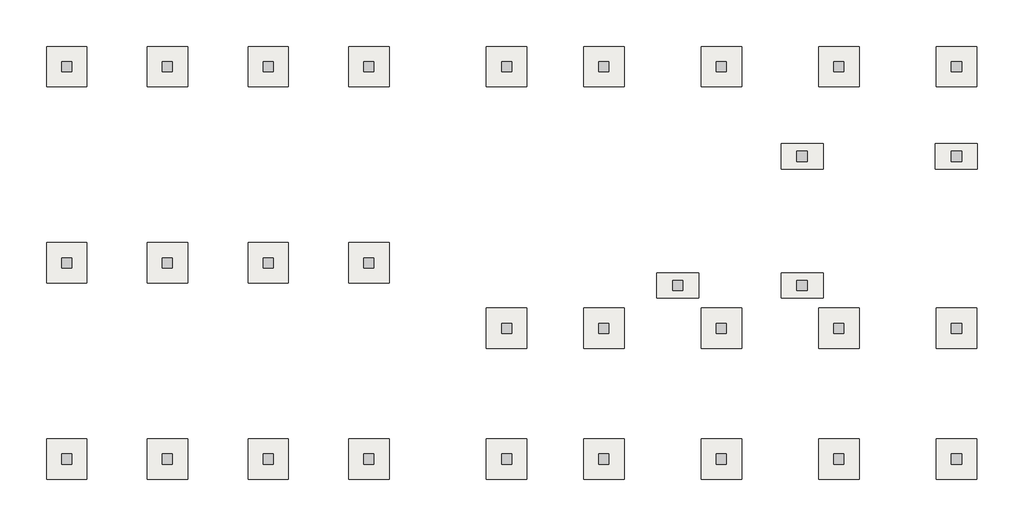
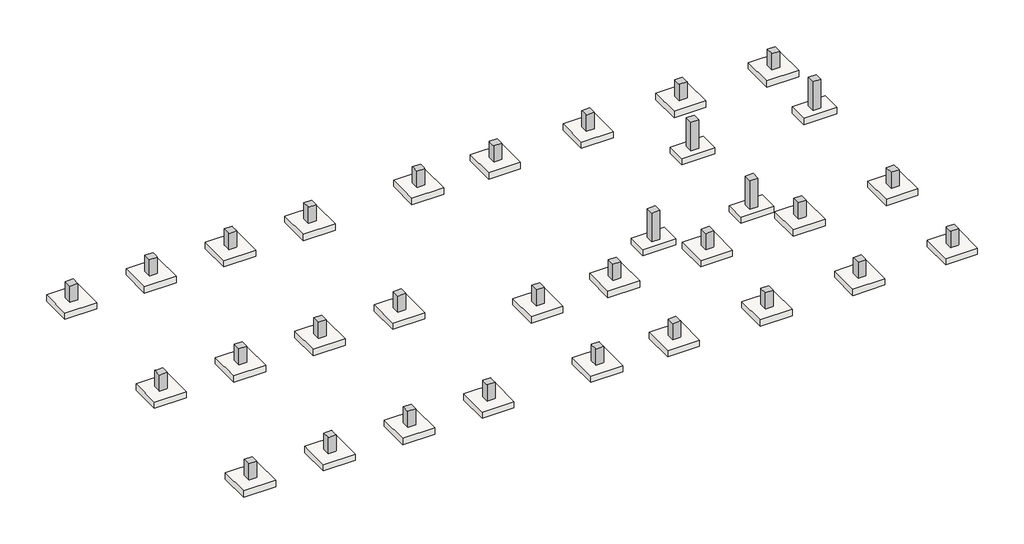
# Not in any storey: 31 columns, 31 slabs.
"""IFC4 building model written with IfcOpenShell, lengths in millimetres."""

import ifcopenshell
import ifcopenshell.guid

model = None  # the IFC model being written
_history = None  # IfcOwnerHistory: only IFC2X3 demands one
_inside = {}  # id of a spatial element -> (the spatial element, [elements in it])
_under = {}  # id of a project, library or spatial element -> (it, [spatial elements below it])
_declared = {}  # id of a project -> (the project, [libraries it declares])
_typed = {}  # id of a type object -> (the type object, [elements of that type])
_made_of = {}  # id of a material, layer set ... -> (it, [elements and type objects made of it])


def new_model(schema):
    """Start an empty IFC model of exactly this schema.

    Asked for "IFC4X3", IfcOpenShell would pick the latest addendum, in which some entities
    have other attributes; the version numbers below select the first issue.
    IFC2X3 requires an IfcOwnerHistory on every rooted entity: one is made here for all.
    """
    global model, _history
    if schema == "IFC4X3":
        model = ifcopenshell.file(schema_version=(4, 3, 0, 0))
    else:
        model = ifcopenshell.file(schema=schema)
    _inside.clear()
    _under.clear()
    _declared.clear()
    _typed.clear()
    _made_of.clear()
    _history = None
    if model.schema == "IFC2X3":
        org = make("IfcOrganization", Name="unknown")
        user = make(
            "IfcPersonAndOrganization",
            ThePerson=make("IfcPerson", FamilyName="unknown"),
            TheOrganization=org,
        )
        app = make(
            "IfcApplication",
            ApplicationDeveloper=org,
            Version="unknown",
            ApplicationFullName="unknown",
            ApplicationIdentifier="unknown",
        )
        _history = make(
            "IfcOwnerHistory",
            OwningUser=user,
            OwningApplication=app,
            ChangeAction="ADDED",
            CreationDate=0,
        )
    return model


def make(cls, **values):
    """One entity of the class cls with the attributes given. An attribute that is None is left unset."""
    return model.create_entity(
        cls, **{name: value for name, value in values.items() if value is not None}
    )


def rooted(cls, **values):
    """An entity with a GlobalId (a new one), such as an element, a storey or a relation."""
    return make(cls, GlobalId=ifcopenshell.guid.new(), OwnerHistory=_history, **values)


def si_unit(unit_type, name, prefix=None):
    """IfcSIUnit, for example si_unit("LENGTHUNIT", "METRE", prefix="MILLI")."""
    return make("IfcSIUnit", UnitType=unit_type, Prefix=prefix, Name=name)


def assignment(units):
    """IfcUnitAssignment: the units of a project."""
    return None if units is None else make("IfcUnitAssignment", Units=units)


def point(xyz):
    """IfcCartesianPoint."""
    return None if xyz is None else make("IfcCartesianPoint", Coordinates=xyz)


def direction(xyz):
    """IfcDirection."""
    return None if xyz is None else make("IfcDirection", DirectionRatios=xyz)


def frame(location, z_axis=None, x_axis=None):
    """IfcAxis2Placement3D, a coordinate frame: its origin and axes. An axis left out is left unset."""
    return make(
        "IfcAxis2Placement3D",
        Location=point(location),
        Axis=direction(z_axis),
        RefDirection=direction(x_axis),
    )


def origin():
    """The frame at (0, 0, 0) with its axes left unset."""
    return frame((0.0, 0.0, 0.0))


def place(relative_to, where):
    """IfcLocalPlacement: puts the frame where relative to a parent placement (None: the world)."""
    return make(
        "IfcLocalPlacement", PlacementRelTo=relative_to, RelativePlacement=where
    )


def context(
    kind, dimensions, precision=None, world=None, true_north=None, identifier=None
):
    """IfcGeometricRepresentationContext, for example the 3D "Model" context."""
    return make(
        "IfcGeometricRepresentationContext",
        ContextIdentifier=identifier,
        ContextType=kind,
        CoordinateSpaceDimension=dimensions,
        Precision=precision,
        WorldCoordinateSystem=world,
        TrueNorth=true_north,
    )


def project(units=None, contexts=None):
    """IfcProject with its units and contexts."""
    return rooted(
        "IfcProject",
        Name="project",
        RepresentationContexts=contexts,
        UnitsInContext=assignment(units),
    )


def spatial(cls, under=None, at=None, **own):
    """A site, building, storey or space (cls), placed at a placement, below another one or the project."""
    s = rooted(cls, ObjectPlacement=at, **own)
    if under is not None:
        _under.setdefault(under.id(), (under, []))[1].append(s)
    return s


def polyline(points):
    """IfcPolyline through the points."""
    return make("IfcPolyline", Points=[point(p) for p in points])


def outline(outer, holes=None, kind="AREA"):
    """IfcArbitraryClosedProfileDef: a profile drawn as a closed curve; with holes, ...WithVoids."""
    if holes is None:
        return make("IfcArbitraryClosedProfileDef", ProfileType=kind, OuterCurve=outer)
    return make(
        "IfcArbitraryProfileDefWithVoids",
        ProfileType=kind,
        OuterCurve=outer,
        InnerCurves=holes,
    )


def extrude(swept, where, along, depth):
    """IfcExtrudedAreaSolid: the profile swept, set in the frame where, extruded along a direction by depth."""
    return make(
        "IfcExtrudedAreaSolid",
        SweptArea=swept,
        Position=where,
        ExtrudedDirection=direction(along),
        Depth=depth,
    )


def faces_of(points, faces, orient=None, outer=None):
    """IfcFace entities. A face is a list of loops; a loop is a list of indices into points, from 0.

    orient and outer hold one flag for each loop. By default every Orientation is true, the
    first loop of a face is its IfcFaceOuterBound and the others are IfcFaceBound.
    """
    made = []
    for i, loops in enumerate(faces):
        bounds = []
        for j, loop in enumerate(loops):
            is_outer = j == 0 if outer is None else outer[i][j]
            bounds.append(
                make(
                    "IfcFaceOuterBound" if is_outer else "IfcFaceBound",
                    Bound=make("IfcPolyLoop", Polygon=[points[k] for k in loop]),
                    Orientation=True if orient is None else orient[i][j],
                )
            )
        made.append(make("IfcFace", Bounds=bounds))
    return made


def faceted_brep(points, faces, orient=None, outer=None, voids=None):
    """IfcFacetedBrep: a solid bounded by flat faces; with voids (closed shells), ...WithVoids."""
    shared = [point(p) for p in points]
    hull = make("IfcClosedShell", CfsFaces=faces_of(shared, faces, orient, outer))
    if voids is None:
        return make("IfcFacetedBrep", Outer=hull)
    return make(
        "IfcFacetedBrepWithVoids",
        Outer=hull,
        Voids=[
            make(cls, CfsFaces=faces_of(shared, fs, o, b)) for cls, fs, o, b in voids
        ],
    )


def shape(context_of_items, identifier, shape_type, items):
    """IfcShapeRepresentation: the items that make up one representation, for example the "Body"."""
    return make(
        "IfcShapeRepresentation",
        ContextOfItems=context_of_items,
        RepresentationIdentifier=identifier,
        RepresentationType=shape_type,
        Items=items,
    )


def source(mapping_origin, context_of_items, identifier, shape_type, items):
    """IfcRepresentationMap: a shape defined once, which mapped items show again and again."""
    return make(
        "IfcRepresentationMap",
        MappingOrigin=mapping_origin,
        MappedRepresentation=shape(context_of_items, identifier, shape_type, items),
    )


def transform(
    local_origin,
    x_axis=None,
    y_axis=None,
    z_axis=None,
    scale=None,
    scale2=None,
    scale3=None,
    uniform=True,
):
    """IfcCartesianTransformationOperator3D, or its non-uniform kind. x_axis, y_axis, z_axis: its Axis1, 2, 3."""
    if uniform:
        return make(
            "IfcCartesianTransformationOperator3D",
            Axis1=direction(x_axis),
            Axis2=direction(y_axis),
            LocalOrigin=point(local_origin),
            Scale=scale,
            Axis3=direction(z_axis),
        )
    return make(
        "IfcCartesianTransformationOperator3DnonUniform",
        Axis1=direction(x_axis),
        Axis2=direction(y_axis),
        LocalOrigin=point(local_origin),
        Scale=scale,
        Axis3=direction(z_axis),
        Scale2=scale2,
        Scale3=scale3,
    )


def mapped(mapping_source, mapping_target):
    """IfcMappedItem: shows the shape of a source again, moved by a transform."""
    return make(
        "IfcMappedItem", MappingSource=mapping_source, MappingTarget=mapping_target
    )


def made_of(thing, what):
    """Note that an element or type object is made of a material, layer set ...; save() writes the relation."""
    if what is not None:
        _made_of.setdefault(what.id(), (what, []))[1].append(thing)
    return thing


def element(
    cls,
    number,
    at=None,
    inside=None,
    cuts=None,
    type_object=None,
    material=None,
    context=None,
    identifier="Body",
    shape_type=None,
    held_by="IfcProductDefinitionShape",
    body=None,
    shapes=None,
    **own,
):
    """One element of the class cls, such as IfcWall. Its Tag is "e" and its number.

    at: its placement. inside: the storey or other place that contains it. cuts: it is an
    opening in that element (IfcRelVoidsElement). A single representation is given by context,
    identifier, shape_type and body (its items); several are given by shapes. held_by: the class
    of the entity that holds the representations. save() writes the other relations.
    """
    e = rooted(cls, Tag="e%d" % number, ObjectPlacement=at, **own)
    if body is not None:
        shapes = [shape(context, identifier, shape_type, body)]
    if shapes is not None:
        e.Representation = make(held_by, Representations=shapes)
    if inside is not None:
        _inside.setdefault(inside.id(), (inside, []))[1].append(e)
    if cuts is not None:
        rooted(
            "IfcRelVoidsElement", RelatingBuildingElement=cuts, RelatedOpeningElement=e
        )
    if type_object is not None:
        _typed.setdefault(type_object.id(), (type_object, []))[1].append(e)
    return made_of(e, material)


def aggregate(whole, parts):
    """IfcRelAggregates: a whole, such as a stair, and the parts it consists of."""
    return rooted("IfcRelAggregates", RelatingObject=whole, RelatedObjects=parts)


def save(model, path):
    """Write the relations noted so far, then the file.

    IfcRelAggregates (storeys below a building ...), IfcRelContainedInSpatialStructure (elements
    in a storey), IfcRelDefinesByType, IfcRelAssociatesMaterial and IfcRelDeclares: one each for
    every whole, place, type object, material and project.
    """
    for whole, parts in _under.values():
        aggregate(whole, parts)
    for where, things in _inside.values():
        rooted(
            "IfcRelContainedInSpatialStructure",
            RelatedElements=things,
            RelatingStructure=where,
        )
    for kind, things in _typed.values():
        rooted("IfcRelDefinesByType", RelatedObjects=things, RelatingType=kind)
    for what, things in _made_of.values():
        rooted("IfcRelAssociatesMaterial", RelatedObjects=things, RelatingMaterial=what)
    for by, libraries in _declared.values():
        rooted("IfcRelDeclares", RelatingContext=by, RelatedDefinitions=libraries)
    model.write(path)


def ft211_footing_rectangular_r1_5fe39465(model_context):
    return source(origin(), model_context, "Body", "SweptSolid", [
        extrude(outline(polyline([(1200.0, 1200.0), (1200.0, -1200.0), (-1200.0, -1200.0), (-1200.0, 1200.0), (1200.0, 1200.0)])), frame((0.0, 0.0, -500.0), z_axis=(0.0, 0.0, 1.0), x_axis=(1.0, 0.0, 0.0)), (0.0, 0.0, 1.0), 500.0),
    ])


def ft211_footing_rectangular_r1_907a7f09(model_context):
    return source(origin(), model_context, "Body", "SweptSolid", [
        extrude(outline(polyline([(1250.0, 750.0), (1250.0, -750.0), (-1250.0, -750.0), (-1250.0, 750.0), (1250.0, 750.0)])), frame((0.0, 0.0, -500.0), z_axis=(0.0, 0.0, 1.0), x_axis=(1.0, 0.0, 0.0)), (0.0, 0.0, 1.0), 500.0),
    ])


model = new_model("IFC4")

# Units and contexts
model_context = context("Model", 3, world=origin())
ifc_project = project(units=[si_unit("LENGTHUNIT", "METRE", prefix="MILLI")], contexts=[model_context])

# Site, building
site = spatial("IfcSite", under=ifc_project)
building = spatial("IfcBuilding", under=site)

# Columns
placement = place(None, origin())
element("IfcColumn", 1, ObjectType="RC_Column_Rectangular : H_SC_ACC_UG PED_W600xL600", at=placement, inside=building, context=model_context, shape_type="Brep", body=[
    faceted_brep([(224.7, 12616.5208589, -1150.0), (224.7, 12016.5208589, -1150.0), (-375.3, 12016.5208589, -1150.0), (-375.3, 12616.5208589, -1150.0), (224.7, 12616.5208589, 150.0), (224.7, 12016.5208589, 150.0), (-375.3, 12016.5208589, 150.0), (-375.3, 12616.5208589, 150.0), (-275.3, 12616.5208589, 150.0), (124.7, 12616.5208589, 150.0)], [[[0, 1, 2, 3]], [[4, 5, 1, 0]], [[5, 6, 2, 1]], [[6, 7, 3, 2]], [[7, 8, 9, 4, 0, 3]], [[4, 9, 8, 7, 6, 5]]]),
])
element("IfcColumn", 2, ObjectType="RC_Column_Rectangular : H_SC_ACC_UG PED_W600xL600", at=placement, inside=building, context=model_context, shape_type="SweptSolid", body=[
    extrude(outline(polyline([(6224.7, 12616.5208589), (6224.7, 12016.5208589), (5624.7, 12016.5208589), (5624.7, 12616.5208589), (6224.7, 12616.5208589)])), frame((0.0, 0.0, -1150.0), z_axis=(0.0, 0.0, 1.0), x_axis=(1.0, 0.0, 0.0)), (0.0, 0.0, 1.0), 1300.0),
])
element("IfcColumn", 3, ObjectType="RC_Column_Rectangular : H_SC_ACC_UG PED_W600xL600", at=placement, inside=building, context=model_context, shape_type="SweptSolid", body=[
    extrude(outline(polyline([(12224.7, 12616.5208589), (12224.7, 12016.5208589), (11624.7, 12016.5208589), (11624.7, 12616.5208589), (12224.7, 12616.5208589)])), frame((0.0, 0.0, -1150.0), z_axis=(0.0, 0.0, 1.0), x_axis=(1.0, 0.0, 0.0)), (0.0, 0.0, 1.0), 1300.0),
])
element("IfcColumn", 4, ObjectType="RC_Column_Rectangular : H_SC_ACC_UG PED_W600xL600", at=placement, inside=building, context=model_context, shape_type="SweptSolid", body=[
    extrude(outline(polyline([(18224.7, 12616.5208589), (18224.7, 12016.5208589), (17624.7, 12016.5208589), (17624.7, 12616.5208589), (18224.7, 12616.5208589)])), frame((0.0, 0.0, -1150.0), z_axis=(0.0, 0.0, 1.0), x_axis=(1.0, 0.0, 0.0)), (0.0, 0.0, 1.0), 1300.0),
])
element("IfcColumn", 5, ObjectType="RC_Column_Rectangular : H_SC_ACC_UG PED_W600xL600", at=placement, inside=building, context=model_context, shape_type="Brep", body=[
    faceted_brep([(224.7, 24316.5208589, -1150.0), (224.7, 23716.5208589, -1150.0), (-375.3, 23716.5208589, -1150.0), (-375.3, 24316.5208589, -1150.0), (224.7, 24316.5208589, 150.0), (224.7, 23716.5208589, 150.0), (124.7, 23716.5208589, 150.0), (-275.3, 23716.5208589, 150.0), (-375.3, 23716.5208589, 150.0), (-375.3, 24316.5208589, 150.0)], [[[0, 1, 2, 3]], [[4, 5, 1, 0]], [[5, 6, 7, 8, 2, 1]], [[8, 9, 3, 2]], [[9, 4, 0, 3]], [[4, 9, 8, 7, 6, 5]]]),
])
element("IfcColumn", 6, ObjectType="RC_Column_Rectangular : H_SC_ACC_UG PED_W600xL600", at=placement, inside=building, context=model_context, shape_type="Brep", body=[
    faceted_brep([(6224.7, 24316.5208589, -1150.0), (6224.7, 23716.5208589, -1150.0), (5624.7, 23716.5208589, -1150.0), (5624.7, 24316.5208589, -1150.0), (6224.7, 24316.5208589, 150.0), (6224.7, 24216.5208589, 150.0), (6224.7, 23816.5208589, 150.0), (6224.7, 23716.5208589, 150.0), (5624.7, 23716.5208589, 150.0), (5624.7, 23816.5208589, 150.0), (5624.7, 24216.5208589, 150.0), (5624.7, 24316.5208589, 150.0)], [[[0, 1, 2, 3]], [[4, 5, 6, 7, 1, 0]], [[7, 8, 2, 1]], [[8, 9, 10, 11, 3, 2]], [[11, 4, 0, 3]], [[4, 11, 10, 9, 8, 7, 6, 5]]]),
])
element("IfcColumn", 7, ObjectType="RC_Column_Rectangular : H_SC_ACC_UG PED_W600xL600", at=placement, inside=building, context=model_context, shape_type="Brep", body=[
    faceted_brep([(12224.7, 24316.5208589, -1150.0), (12224.7, 23716.5208589, -1150.0), (11624.7, 23716.5208589, -1150.0), (11624.7, 24316.5208589, -1150.0), (12224.7, 24316.5208589, 150.0), (12224.7, 24216.5208589, 150.0), (12224.7, 23816.5208589, 150.0), (12224.7, 23716.5208589, 150.0), (11624.7, 23716.5208589, 150.0), (11624.7, 23816.5208589, 150.0), (11624.7, 24216.5208589, 150.0), (11624.7, 24316.5208589, 150.0)], [[[0, 1, 2, 3]], [[4, 5, 6, 7, 1, 0]], [[7, 8, 2, 1]], [[8, 9, 10, 11, 3, 2]], [[11, 4, 0, 3]], [[4, 11, 10, 9, 8, 7, 6, 5]]]),
])
element("IfcColumn", 8, ObjectType="RC_Column_Rectangular : H_SC_ACC_UG PED_W600xL600", at=placement, inside=building, context=model_context, shape_type="Brep", body=[
    faceted_brep([(18224.7, 24316.5208589, -1150.0), (18224.7, 23716.5208589, -1150.0), (17624.7, 23716.5208589, -1150.0), (17624.7, 24316.5208589, -1150.0), (18224.7, 24316.5208589, 150.0), (18224.7, 24216.5208589, 150.0), (18224.7, 23816.5208589, 150.0), (18224.7, 23716.5208589, 150.0), (17624.7, 23716.5208589, 150.0), (17624.7, 23816.5208589, 150.0), (17624.7, 24216.5208589, 150.0), (17624.7, 24316.5208589, 150.0)], [[[0, 1, 2, 3]], [[4, 5, 6, 7, 1, 0]], [[7, 8, 2, 1]], [[8, 9, 10, 11, 3, 2]], [[11, 4, 0, 3]], [[4, 11, 10, 9, 8, 7, 6, 5]]]),
])
element("IfcColumn", 9, ObjectType="RC_Column_Rectangular : H_SC_ACC_UG PED_W600xL600", at=placement, inside=building, context=model_context, shape_type="Brep", body=[
    faceted_brep([(26424.7, 24316.5208589, -1150.0), (26424.7, 23716.5208589, -1150.0), (25824.7, 23716.5208589, -1150.0), (25824.7, 24316.5208589, -1150.0), (26424.7, 24316.5208589, 150.0), (26424.7, 24216.5208589, 150.0), (26424.7, 23816.5208589, 150.0), (26424.7, 23716.5208589, 150.0), (25824.7, 23716.5208589, 150.0), (25824.7, 23816.5208589, 150.0), (25824.7, 24216.5208589, 150.0), (25824.7, 24316.5208589, 150.0)], [[[0, 1, 2, 3]], [[4, 5, 6, 7, 1, 0]], [[7, 8, 2, 1]], [[8, 9, 10, 11, 3, 2]], [[11, 4, 0, 3]], [[4, 11, 10, 9, 8, 7, 6, 5]]]),
])
element("IfcColumn", 10, ObjectType="RC_Column_Rectangular : H_SC_ACC_UG PED_W600xL600", at=placement, inside=building, context=model_context, shape_type="Brep", body=[
    faceted_brep([(32224.7, 24316.5208589, -1150.0), (32224.7, 23716.5208589, -1150.0), (31624.7, 23716.5208589, -1150.0), (31624.7, 24316.5208589, -1150.0), (32224.7, 24316.5208589, 150.0), (32224.7, 24216.5208589, 150.0), (32224.7, 23816.5208589, 150.0), (32224.7, 23716.5208589, 150.0), (31624.7, 23716.5208589, 150.0), (31624.7, 23816.5208589, 150.0), (31624.7, 24216.5208589, 150.0), (31624.7, 24316.5208589, 150.0)], [[[0, 1, 2, 3]], [[4, 5, 6, 7, 1, 0]], [[7, 8, 2, 1]], [[8, 9, 10, 11, 3, 2]], [[11, 4, 0, 3]], [[4, 11, 10, 9, 8, 7, 6, 5]]]),
])
element("IfcColumn", 11, ObjectType="RC_Column_Rectangular : H_SC_ACC_UG PED_W600xL600", at=placement, inside=building, context=model_context, shape_type="Brep", body=[
    faceted_brep([(39224.7, 24316.5208589, -1150.0), (39224.7, 23716.5208589, -1150.0), (38624.7, 23716.5208589, -1150.0), (38624.7, 24316.5208589, -1150.0), (39224.7, 24316.5208589, 150.0), (39224.7, 24216.5208589, 150.0), (39224.7, 23816.5208589, 150.0), (39224.7, 23716.5208589, 150.0), (38624.7, 23716.5208589, 150.0), (38624.7, 23816.5208589, 150.0), (38624.7, 24216.5208589, 150.0), (38624.7, 24316.5208589, 150.0)], [[[0, 1, 2, 3]], [[4, 5, 6, 7, 1, 0]], [[7, 8, 2, 1]], [[8, 9, 10, 11, 3, 2]], [[11, 4, 0, 3]], [[4, 11, 10, 9, 8, 7, 6, 5]]]),
])
element("IfcColumn", 12, ObjectType="RC_Column_Rectangular : H_SC_ACC_UG PED_W600xL600", at=placement, inside=building, context=model_context, shape_type="Brep", body=[
    faceted_brep([(46224.7, 24316.5208589, -1150.0), (46224.7, 23716.5208589, -1150.0), (45624.7, 23716.5208589, -1150.0), (45624.7, 24316.5208589, -1150.0), (46224.7, 24316.5208589, 150.0), (46224.7, 24216.5208589, 150.0), (46224.7, 23816.5208589, 150.0), (46224.7, 23716.5208589, 150.0), (45624.7, 23716.5208589, 150.0), (45624.7, 23816.5208589, 150.0), (45624.7, 24216.5208589, 150.0), (45624.7, 24316.5208589, 150.0)], [[[0, 1, 2, 3]], [[4, 5, 6, 7, 1, 0]], [[7, 8, 2, 1]], [[8, 9, 10, 11, 3, 2]], [[11, 4, 0, 3]], [[4, 11, 10, 9, 8, 7, 6, 5]]]),
])
element("IfcColumn", 13, ObjectType="RC_Column_Rectangular : H_SC_ACC_UG PED_W600xL600", at=placement, inside=building, context=model_context, shape_type="Brep", body=[
    faceted_brep([(53224.7, 24316.5208589, -1150.0), (53224.7, 23716.5208589, -1150.0), (52624.7, 23716.5208589, -1150.0), (52624.7, 24316.5208589, -1150.0), (53224.7, 24316.5208589, 150.0), (53224.7, 23716.5208589, 150.0), (53124.7, 23716.5208589, 150.0), (52724.7, 23716.5208589, 150.0), (52624.7, 23716.5208589, 150.0), (52624.7, 23816.5208589, 150.0), (52624.7, 24216.5208589, 150.0), (52624.7, 24316.5208589, 150.0)], [[[0, 1, 2, 3]], [[4, 5, 1, 0]], [[5, 6, 7, 8, 2, 1]], [[8, 9, 10, 11, 3, 2]], [[11, 4, 0, 3]], [[4, 11, 10, 9, 8, 7, 6, 5]]]),
])
element("IfcColumn", 14, ObjectType="RC_Column_Rectangular : H_SC_ACC_UG PED_W600xL600", at=placement, inside=building, context=model_context, shape_type="SweptSolid", body=[
    extrude(outline(polyline([(26424.7, 8716.5208589), (26424.7, 8116.5208589), (25824.7, 8116.5208589), (25824.7, 8716.5208589), (26424.7, 8716.5208589)])), frame((0.0, 0.0, -1150.0), z_axis=(0.0, 0.0, 1.0), x_axis=(1.0, 0.0, 0.0)), (0.0, 0.0, 1.0), 1300.0),
])
element("IfcColumn", 15, ObjectType="RC_Column_Rectangular : H_SC_ACC_UG PED_W600xL600", at=placement, inside=building, context=model_context, shape_type="SweptSolid", body=[
    extrude(outline(polyline([(32224.7, 8716.5208589), (32224.7, 8116.5208589), (31624.7, 8116.5208589), (31624.7, 8716.5208589), (32224.7, 8716.5208589)])), frame((0.0, 0.0, -1150.0), z_axis=(0.0, 0.0, 1.0), x_axis=(1.0, 0.0, 0.0)), (0.0, 0.0, 1.0), 1300.0),
])
element("IfcColumn", 16, ObjectType="RC_Column_Rectangular : H_SC_ACC_UG PED_W600xL600", at=placement, inside=building, context=model_context, shape_type="SweptSolid", body=[
    extrude(outline(polyline([(39224.7, 8716.5208589), (39224.7, 8116.5208589), (38624.7, 8116.5208589), (38624.7, 8716.5208589), (39224.7, 8716.5208589)])), frame((0.0, 0.0, -1150.0), z_axis=(0.0, 0.0, 1.0), x_axis=(1.0, 0.0, 0.0)), (0.0, 0.0, 1.0), 1300.0),
])
element("IfcColumn", 17, ObjectType="RC_Column_Rectangular : H_SC_ACC_UG PED_W600xL600", at=placement, inside=building, context=model_context, shape_type="SweptSolid", body=[
    extrude(outline(polyline([(46224.7, 8716.5208589), (46224.7, 8116.5208589), (45624.7, 8116.5208589), (45624.7, 8716.5208589), (46224.7, 8716.5208589)])), frame((0.0, 0.0, -1150.0), z_axis=(0.0, 0.0, 1.0), x_axis=(1.0, 0.0, 0.0)), (0.0, 0.0, 1.0), 1300.0),
])
element("IfcColumn", 18, ObjectType="RC_Column_Rectangular : H_SC_ACC_UG PED_W600xL600", at=placement, inside=building, context=model_context, shape_type="Brep", body=[
    faceted_brep([(53224.7, 8716.5208589, -1150.0), (53224.7, 8116.5208589, -1150.0), (52624.7, 8116.5208589, -1150.0), (52624.7, 8716.5208589, -1150.0), (53224.7, 8716.5208589, 150.0), (53224.7, 8116.5208589, 150.0), (53124.7, 8116.5208589, 150.0), (52724.7, 8116.5208589, 150.0), (52624.7, 8116.5208589, 150.0), (52624.7, 8716.5208589, 150.0), (52724.7, 8716.5208589, 150.0), (53124.7, 8716.5208589, 150.0)], [[[0, 1, 2, 3]], [[4, 5, 1, 0]], [[5, 6, 7, 8, 2, 1]], [[8, 9, 3, 2]], [[9, 10, 11, 4, 0, 3]], [[4, 11, 10, 9, 8, 7, 6, 5]]]),
])
element("IfcColumn", 19, ObjectType="RC_Column_Rectangular : H_SC_ACC_UG PED_W600xL600", at=placement, inside=building, context=model_context, shape_type="Brep", body=[
    faceted_brep([(224.7, 916.5208589, -1150.0), (224.7, 316.5208589, -1150.0), (-375.3, 316.5208589, -1150.0), (-375.3, 916.5208589, -1150.0), (224.7, 916.5208589, 150.0), (224.7, 816.5208589, 150.0), (224.7, 416.5208589, 150.0), (224.7, 316.5208589, 150.0), (-375.3, 316.5208589, 150.0), (-375.3, 916.5208589, 150.0), (-275.3, 916.5208589, 150.0), (124.7, 916.5208589, 150.0)], [[[0, 1, 2, 3]], [[4, 5, 6, 7, 1, 0]], [[7, 8, 2, 1]], [[8, 9, 3, 2]], [[9, 10, 11, 4, 0, 3]], [[4, 11, 10, 9, 8, 7, 6, 5]]]),
])
element("IfcColumn", 20, ObjectType="RC_Column_Rectangular : H_SC_ACC_UG PED_W600xL600", at=placement, inside=building, context=model_context, shape_type="Brep", body=[
    faceted_brep([(6224.7, 916.5208589, -1150.0), (6224.7, 316.5208589, -1150.0), (5624.7, 316.5208589, -1150.0), (5624.7, 916.5208589, -1150.0), (6224.7, 916.5208589, 150.0), (6224.7, 816.5208589, 150.0), (6224.7, 416.5208589, 150.0), (6224.7, 316.5208589, 150.0), (5624.7, 316.5208589, 150.0), (5624.7, 416.5208589, 150.0), (5624.7, 816.5208589, 150.0), (5624.7, 916.5208589, 150.0)], [[[0, 1, 2, 3]], [[4, 5, 6, 7, 1, 0]], [[7, 8, 2, 1]], [[8, 9, 10, 11, 3, 2]], [[11, 4, 0, 3]], [[4, 11, 10, 9, 8, 7, 6, 5]]]),
])
element("IfcColumn", 21, ObjectType="RC_Column_Rectangular : H_SC_ACC_UG PED_W600xL600", at=placement, inside=building, context=model_context, shape_type="Brep", body=[
    faceted_brep([(12224.7, 916.5208589, -1150.0), (12224.7, 316.5208589, -1150.0), (11624.7, 316.5208589, -1150.0), (11624.7, 916.5208589, -1150.0), (12224.7, 916.5208589, 150.0), (12224.7, 816.5208589, 150.0), (12224.7, 416.5208589, 150.0), (12224.7, 316.5208589, 150.0), (11624.7, 316.5208589, 150.0), (11624.7, 416.5208589, 150.0), (11624.7, 816.5208589, 150.0), (11624.7, 916.5208589, 150.0)], [[[0, 1, 2, 3]], [[4, 5, 6, 7, 1, 0]], [[7, 8, 2, 1]], [[8, 9, 10, 11, 3, 2]], [[11, 4, 0, 3]], [[4, 11, 10, 9, 8, 7, 6, 5]]]),
])
element("IfcColumn", 22, ObjectType="RC_Column_Rectangular : H_SC_ACC_UG PED_W600xL600", at=placement, inside=building, context=model_context, shape_type="Brep", body=[
    faceted_brep([(18224.7, 916.5208589, -1150.0), (18224.7, 316.5208589, -1150.0), (17624.7, 316.5208589, -1150.0), (17624.7, 916.5208589, -1150.0), (18224.7, 916.5208589, 150.0), (18224.7, 816.5208589, 150.0), (18224.7, 416.5208589, 150.0), (18224.7, 316.5208589, 150.0), (17624.7, 316.5208589, 150.0), (17624.7, 416.5208589, 150.0), (17624.7, 816.5208589, 150.0), (17624.7, 916.5208589, 150.0)], [[[0, 1, 2, 3]], [[4, 5, 6, 7, 1, 0]], [[7, 8, 2, 1]], [[8, 9, 10, 11, 3, 2]], [[11, 4, 0, 3]], [[4, 11, 10, 9, 8, 7, 6, 5]]]),
])
element("IfcColumn", 23, ObjectType="RC_Column_Rectangular : H_SC_ACC_UG PED_W600xL600", at=placement, inside=building, context=model_context, shape_type="Brep", body=[
    faceted_brep([(26424.7, 916.5208589, -1150.0), (26424.7, 316.5208589, -1150.0), (25824.7, 316.5208589, -1150.0), (25824.7, 916.5208589, -1150.0), (26424.7, 916.5208589, 150.0), (26424.7, 816.5208589, 150.0), (26424.7, 416.5208589, 150.0), (26424.7, 316.5208589, 150.0), (25824.7, 316.5208589, 150.0), (25824.7, 416.5208589, 150.0), (25824.7, 816.5208589, 150.0), (25824.7, 916.5208589, 150.0)], [[[0, 1, 2, 3]], [[4, 5, 6, 7, 1, 0]], [[7, 8, 2, 1]], [[8, 9, 10, 11, 3, 2]], [[11, 4, 0, 3]], [[4, 11, 10, 9, 8, 7, 6, 5]]]),
])
element("IfcColumn", 24, ObjectType="RC_Column_Rectangular : H_SC_ACC_UG PED_W600xL600", at=placement, inside=building, context=model_context, shape_type="Brep", body=[
    faceted_brep([(32224.7, 916.5208589, -1150.0), (32224.7, 316.5208589, -1150.0), (31624.7, 316.5208589, -1150.0), (31624.7, 916.5208589, -1150.0), (32224.7, 916.5208589, 150.0), (32224.7, 816.5208589, 150.0), (32224.7, 416.5208589, 150.0), (32224.7, 316.5208589, 150.0), (31624.7, 316.5208589, 150.0), (31624.7, 416.5208589, 150.0), (31624.7, 816.5208589, 150.0), (31624.7, 916.5208589, 150.0)], [[[0, 1, 2, 3]], [[4, 5, 6, 7, 1, 0]], [[7, 8, 2, 1]], [[8, 9, 10, 11, 3, 2]], [[11, 4, 0, 3]], [[4, 11, 10, 9, 8, 7, 6, 5]]]),
])
element("IfcColumn", 25, ObjectType="RC_Column_Rectangular : H_SC_ACC_UG PED_W600xL600", at=placement, inside=building, context=model_context, shape_type="Brep", body=[
    faceted_brep([(39224.7, 916.5208589, -1150.0), (39224.7, 316.5208589, -1150.0), (38624.7, 316.5208589, -1150.0), (38624.7, 916.5208589, -1150.0), (39224.7, 916.5208589, 150.0), (39224.7, 816.5208589, 150.0), (39224.7, 416.5208589, 150.0), (39224.7, 316.5208589, 150.0), (38624.7, 316.5208589, 150.0), (38624.7, 416.5208589, 150.0), (38624.7, 816.5208589, 150.0), (38624.7, 916.5208589, 150.0)], [[[0, 1, 2, 3]], [[4, 5, 6, 7, 1, 0]], [[7, 8, 2, 1]], [[8, 9, 10, 11, 3, 2]], [[11, 4, 0, 3]], [[4, 11, 10, 9, 8, 7, 6, 5]]]),
])
element("IfcColumn", 26, ObjectType="RC_Column_Rectangular : H_SC_ACC_UG PED_W600xL600", at=placement, inside=building, context=model_context, shape_type="Brep", body=[
    faceted_brep([(46224.7, 916.5208589, -1150.0), (46224.7, 316.5208589, -1150.0), (45624.7, 316.5208589, -1150.0), (45624.7, 916.5208589, -1150.0), (46224.7, 916.5208589, 150.0), (46224.7, 816.5208589, 150.0), (46224.7, 416.5208589, 150.0), (46224.7, 316.5208589, 150.0), (45624.7, 316.5208589, 150.0), (45624.7, 416.5208589, 150.0), (45624.7, 816.5208589, 150.0), (45624.7, 916.5208589, 150.0)], [[[0, 1, 2, 3]], [[4, 5, 6, 7, 1, 0]], [[7, 8, 2, 1]], [[8, 9, 10, 11, 3, 2]], [[11, 4, 0, 3]], [[4, 11, 10, 9, 8, 7, 6, 5]]]),
])
element("IfcColumn", 27, ObjectType="RC_Column_Rectangular : H_SC_ACC_UG PED_W600xL600", at=placement, inside=building, context=model_context, shape_type="Brep", body=[
    faceted_brep([(53224.7, 916.5208589, -1150.0), (53224.7, 316.5208589, -1150.0), (52624.7, 316.5208589, -1150.0), (52624.7, 916.5208589, -1150.0), (53224.7, 916.5208589, 150.0), (53224.7, 316.5208589, 150.0), (52624.7, 316.5208589, 150.0), (52624.7, 416.5208589, 150.0), (52624.7, 816.5208589, 150.0), (52624.7, 916.5208589, 150.0), (52724.7, 916.5208589, 150.0), (53124.7, 916.5208589, 150.0)], [[[0, 1, 2, 3]], [[4, 5, 1, 0]], [[5, 6, 2, 1]], [[6, 7, 8, 9, 3, 2]], [[9, 10, 11, 4, 0, 3]], [[4, 11, 10, 9, 8, 7, 6, 5]]]),
])
element("IfcColumn", 28, ObjectType="RC_Column_Rectangular : H_SC_ACC_UG PED_W600xL600", at=placement, inside=building, context=model_context, shape_type="SweptSolid", body=[
    extrude(outline(polyline([(36624.7, 11266.5208589), (36624.7, 10666.5208589), (36024.7, 10666.5208589), (36024.7, 11266.5208589), (36624.7, 11266.5208589)])), frame((0.0, 0.0, -1150.0), z_axis=(0.0, 0.0, 1.0), x_axis=(1.0, 0.0, 0.0)), (0.0, 0.0, 1.0), 2300.0),
])
element("IfcColumn", 29, ObjectType="RC_Column_Rectangular : H_SC_ACC_UG PED_W600xL600", at=placement, inside=building, context=model_context, shape_type="SweptSolid", body=[
    extrude(outline(polyline([(44024.7, 11266.5208589), (44024.7, 10666.5208589), (43424.7, 10666.5208589), (43424.7, 11266.5208589), (44024.7, 11266.5208589)])), frame((0.0, 0.0, -1150.0), z_axis=(0.0, 0.0, 1.0), x_axis=(1.0, 0.0, 0.0)), (0.0, 0.0, 1.0), 2300.0),
])
element("IfcColumn", 30, ObjectType="RC_Column_Rectangular : H_SC_ACC_UG PED_W600xL600", at=placement, inside=building, context=model_context, shape_type="SweptSolid", body=[
    extrude(outline(polyline([(44024.7, 18966.5208589), (44024.7, 18366.5208589), (43424.7, 18366.5208589), (43424.7, 18966.5208589), (44024.7, 18966.5208589)])), frame((0.0, 0.0, -1150.0), z_axis=(0.0, 0.0, 1.0), x_axis=(1.0, 0.0, 0.0)), (0.0, 0.0, 1.0), 2300.0),
])
element("IfcColumn", 31, ObjectType="RC_Column_Rectangular : H_SC_ACC_UG PED_W600xL600", at=placement, inside=building, context=model_context, shape_type="SweptSolid", body=[
    extrude(outline(polyline([(53224.7, 18966.5208589), (53224.7, 18366.5208589), (52624.7, 18366.5208589), (52624.7, 18966.5208589), (53224.7, 18966.5208589)])), frame((0.0, 0.0, -1150.0), z_axis=(0.0, 0.0, 1.0), x_axis=(1.0, 0.0, 0.0)), (0.0, 0.0, 1.0), 2300.0),
])

# Slabs
ft211_footing_rectangular_r1_shape = ft211_footing_rectangular_r1_5fe39465(model_context)
element("IfcSlab", 32, ObjectType="FT211-Footing-Rectangular_R1 : H_SF_ACF_W2400xL2400xT500_Bitumen", at=placement, inside=building, context=model_context, shape_type="MappedRepresentation", body=[
    mapped(ft211_footing_rectangular_r1_shape, transform((-75.3, 12316.5208589, -1150.0), x_axis=(1.0, 0.0, 0.0), y_axis=(0.0, 1.0, 0.0), z_axis=(0.0, 0.0, 1.0))),
])
element("IfcSlab", 33, ObjectType="FT211-Footing-Rectangular_R1 : H_SF_ACF_W2400xL2400xT500_Bitumen", at=placement, inside=building, context=model_context, shape_type="MappedRepresentation", body=[
    mapped(ft211_footing_rectangular_r1_shape, transform((5924.7, 12316.5208589, -1150.0), x_axis=(1.0, 0.0, 0.0), y_axis=(0.0, 1.0, 0.0), z_axis=(0.0, 0.0, 1.0))),
])
element("IfcSlab", 34, ObjectType="FT211-Footing-Rectangular_R1 : H_SF_ACF_W2400xL2400xT500_Bitumen", at=placement, inside=building, context=model_context, shape_type="MappedRepresentation", body=[
    mapped(ft211_footing_rectangular_r1_shape, transform((11924.7, 12316.5208589, -1150.0), x_axis=(1.0, 0.0, 0.0), y_axis=(0.0, 1.0, 0.0), z_axis=(0.0, 0.0, 1.0))),
])
element("IfcSlab", 35, ObjectType="FT211-Footing-Rectangular_R1 : H_SF_ACF_W2400xL2400xT500_Bitumen", at=placement, inside=building, context=model_context, shape_type="MappedRepresentation", body=[
    mapped(ft211_footing_rectangular_r1_shape, transform((17924.7, 12316.5208589, -1150.0), x_axis=(1.0, 0.0, 0.0), y_axis=(0.0, 1.0, 0.0), z_axis=(0.0, 0.0, 1.0))),
])
element("IfcSlab", 36, ObjectType="FT211-Footing-Rectangular_R1 : H_SF_ACF_W2400xL2400xT500_Bitumen", at=placement, inside=building, context=model_context, shape_type="MappedRepresentation", body=[
    mapped(ft211_footing_rectangular_r1_shape, transform((-75.3, 24016.5208589, -1150.0), x_axis=(1.0, 0.0, 0.0), y_axis=(0.0, 1.0, 0.0), z_axis=(0.0, 0.0, 1.0))),
])
element("IfcSlab", 37, ObjectType="FT211-Footing-Rectangular_R1 : H_SF_ACF_W2400xL2400xT500_Bitumen", at=placement, inside=building, context=model_context, shape_type="MappedRepresentation", body=[
    mapped(ft211_footing_rectangular_r1_shape, transform((5924.7, 24016.5208589, -1150.0), x_axis=(1.0, 0.0, 0.0), y_axis=(0.0, 1.0, 0.0), z_axis=(0.0, 0.0, 1.0))),
])
element("IfcSlab", 38, ObjectType="FT211-Footing-Rectangular_R1 : H_SF_ACF_W2400xL2400xT500_Bitumen", at=placement, inside=building, context=model_context, shape_type="MappedRepresentation", body=[
    mapped(ft211_footing_rectangular_r1_shape, transform((11924.7, 24016.5208589, -1150.0), x_axis=(1.0, 0.0, 0.0), y_axis=(0.0, 1.0, 0.0), z_axis=(0.0, 0.0, 1.0))),
])
element("IfcSlab", 39, ObjectType="FT211-Footing-Rectangular_R1 : H_SF_ACF_W2400xL2400xT500_Bitumen", at=placement, inside=building, context=model_context, shape_type="MappedRepresentation", body=[
    mapped(ft211_footing_rectangular_r1_shape, transform((17924.7, 24016.5208589, -1150.0), x_axis=(1.0, 0.0, 0.0), y_axis=(0.0, 1.0, 0.0), z_axis=(0.0, 0.0, 1.0))),
])
element("IfcSlab", 40, ObjectType="FT211-Footing-Rectangular_R1 : H_SF_ACF_W2400xL2400xT500_Bitumen", at=placement, inside=building, context=model_context, shape_type="MappedRepresentation", body=[
    mapped(ft211_footing_rectangular_r1_shape, transform((26124.7, 24016.5208589, -1150.0), x_axis=(1.0, 0.0, 0.0), y_axis=(0.0, 1.0, 0.0), z_axis=(0.0, 0.0, 1.0))),
])
element("IfcSlab", 41, ObjectType="FT211-Footing-Rectangular_R1 : H_SF_ACF_W2400xL2400xT500_Bitumen", at=placement, inside=building, context=model_context, shape_type="MappedRepresentation", body=[
    mapped(ft211_footing_rectangular_r1_shape, transform((31924.7, 24016.5208589, -1150.0), x_axis=(1.0, 0.0, 0.0), y_axis=(0.0, 1.0, 0.0), z_axis=(0.0, 0.0, 1.0))),
])
element("IfcSlab", 42, ObjectType="FT211-Footing-Rectangular_R1 : H_SF_ACF_W2400xL2400xT500_Bitumen", at=placement, inside=building, context=model_context, shape_type="MappedRepresentation", body=[
    mapped(ft211_footing_rectangular_r1_shape, transform((38924.7, 24016.5208589, -1150.0), x_axis=(1.0, 0.0, 0.0), y_axis=(0.0, 1.0, 0.0), z_axis=(0.0, 0.0, 1.0))),
])
element("IfcSlab", 43, ObjectType="FT211-Footing-Rectangular_R1 : H_SF_ACF_W2400xL2400xT500_Bitumen", at=placement, inside=building, context=model_context, shape_type="MappedRepresentation", body=[
    mapped(ft211_footing_rectangular_r1_shape, transform((45924.7, 24016.5208589, -1150.0), x_axis=(1.0, 0.0, 0.0), y_axis=(0.0, 1.0, 0.0), z_axis=(0.0, 0.0, 1.0))),
])
element("IfcSlab", 44, ObjectType="FT211-Footing-Rectangular_R1 : H_SF_ACF_W2400xL2400xT500_Bitumen", at=placement, inside=building, context=model_context, shape_type="MappedRepresentation", body=[
    mapped(ft211_footing_rectangular_r1_shape, transform((52924.7, 24016.5208589, -1150.0), x_axis=(1.0, 0.0, 0.0), y_axis=(0.0, 1.0, 0.0), z_axis=(0.0, 0.0, 1.0))),
])
element("IfcSlab", 45, ObjectType="FT211-Footing-Rectangular_R1 : H_SF_ACF_W2400xL2400xT500_Bitumen", at=placement, inside=building, context=model_context, shape_type="MappedRepresentation", body=[
    mapped(ft211_footing_rectangular_r1_shape, transform((26124.7, 8416.5208589, -1150.0), x_axis=(1.0, 0.0, 0.0), y_axis=(0.0, 1.0, 0.0), z_axis=(0.0, 0.0, 1.0))),
])
element("IfcSlab", 46, ObjectType="FT211-Footing-Rectangular_R1 : H_SF_ACF_W2400xL2400xT500_Bitumen", at=placement, inside=building, context=model_context, shape_type="MappedRepresentation", body=[
    mapped(ft211_footing_rectangular_r1_shape, transform((31924.7, 8416.5208589, -1150.0), x_axis=(1.0, 0.0, 0.0), y_axis=(0.0, 1.0, 0.0), z_axis=(0.0, 0.0, 1.0))),
])
element("IfcSlab", 47, ObjectType="FT211-Footing-Rectangular_R1 : H_SF_ACF_W2400xL2400xT500_Bitumen", at=placement, inside=building, context=model_context, shape_type="MappedRepresentation", body=[
    mapped(ft211_footing_rectangular_r1_shape, transform((38924.7, 8416.5208589, -1150.0), x_axis=(1.0, 0.0, 0.0), y_axis=(0.0, 1.0, 0.0), z_axis=(0.0, 0.0, 1.0))),
])
element("IfcSlab", 48, ObjectType="FT211-Footing-Rectangular_R1 : H_SF_ACF_W2400xL2400xT500_Bitumen", at=placement, inside=building, context=model_context, shape_type="MappedRepresentation", body=[
    mapped(ft211_footing_rectangular_r1_shape, transform((45924.7, 8416.5208589, -1150.0), x_axis=(1.0, 0.0, 0.0), y_axis=(0.0, 1.0, 0.0), z_axis=(0.0, 0.0, 1.0))),
])
element("IfcSlab", 49, ObjectType="FT211-Footing-Rectangular_R1 : H_SF_ACF_W2400xL2400xT500_Bitumen", at=placement, inside=building, context=model_context, shape_type="MappedRepresentation", body=[
    mapped(ft211_footing_rectangular_r1_shape, transform((52924.7, 8416.5208589, -1150.0), x_axis=(1.0, 0.0, 0.0), y_axis=(0.0, 1.0, 0.0), z_axis=(0.0, 0.0, 1.0))),
])
element("IfcSlab", 50, ObjectType="FT211-Footing-Rectangular_R1 : H_SF_ACF_W2400xL2400xT500_Bitumen", at=placement, inside=building, context=model_context, shape_type="MappedRepresentation", body=[
    mapped(ft211_footing_rectangular_r1_shape, transform((-75.3, 616.5208589, -1150.0), x_axis=(1.0, 0.0, 0.0), y_axis=(0.0, 1.0, 0.0), z_axis=(0.0, 0.0, 1.0))),
])
element("IfcSlab", 51, ObjectType="FT211-Footing-Rectangular_R1 : H_SF_ACF_W2400xL2400xT500_Bitumen", at=placement, inside=building, context=model_context, shape_type="MappedRepresentation", body=[
    mapped(ft211_footing_rectangular_r1_shape, transform((5924.7, 616.5208589, -1150.0), x_axis=(1.0, 0.0, 0.0), y_axis=(0.0, 1.0, 0.0), z_axis=(0.0, 0.0, 1.0))),
])
element("IfcSlab", 52, ObjectType="FT211-Footing-Rectangular_R1 : H_SF_ACF_W2400xL2400xT500_Bitumen", at=placement, inside=building, context=model_context, shape_type="MappedRepresentation", body=[
    mapped(ft211_footing_rectangular_r1_shape, transform((11924.7, 616.5208589, -1150.0), x_axis=(1.0, 0.0, 0.0), y_axis=(0.0, 1.0, 0.0), z_axis=(0.0, 0.0, 1.0))),
])
element("IfcSlab", 53, ObjectType="FT211-Footing-Rectangular_R1 : H_SF_ACF_W2400xL2400xT500_Bitumen", at=placement, inside=building, context=model_context, shape_type="MappedRepresentation", body=[
    mapped(ft211_footing_rectangular_r1_shape, transform((17924.7, 616.5208589, -1150.0), x_axis=(1.0, 0.0, 0.0), y_axis=(0.0, 1.0, 0.0), z_axis=(0.0, 0.0, 1.0))),
])
element("IfcSlab", 54, ObjectType="FT211-Footing-Rectangular_R1 : H_SF_ACF_W2400xL2400xT500_Bitumen", at=placement, inside=building, context=model_context, shape_type="MappedRepresentation", body=[
    mapped(ft211_footing_rectangular_r1_shape, transform((26124.7, 616.5208589, -1150.0), x_axis=(1.0, 0.0, 0.0), y_axis=(0.0, 1.0, 0.0), z_axis=(0.0, 0.0, 1.0))),
])
element("IfcSlab", 55, ObjectType="FT211-Footing-Rectangular_R1 : H_SF_ACF_W2400xL2400xT500_Bitumen", at=placement, inside=building, context=model_context, shape_type="MappedRepresentation", body=[
    mapped(ft211_footing_rectangular_r1_shape, transform((31924.7, 616.5208589, -1150.0), x_axis=(1.0, 0.0, 0.0), y_axis=(0.0, 1.0, 0.0), z_axis=(0.0, 0.0, 1.0))),
])
element("IfcSlab", 56, ObjectType="FT211-Footing-Rectangular_R1 : H_SF_ACF_W2400xL2400xT500_Bitumen", at=placement, inside=building, context=model_context, shape_type="MappedRepresentation", body=[
    mapped(ft211_footing_rectangular_r1_shape, transform((38924.7, 616.5208589, -1150.0), x_axis=(1.0, 0.0, 0.0), y_axis=(0.0, 1.0, 0.0), z_axis=(0.0, 0.0, 1.0))),
])
element("IfcSlab", 57, ObjectType="FT211-Footing-Rectangular_R1 : H_SF_ACF_W2400xL2400xT500_Bitumen", at=placement, inside=building, context=model_context, shape_type="MappedRepresentation", body=[
    mapped(ft211_footing_rectangular_r1_shape, transform((45924.7, 616.5208589, -1150.0), x_axis=(1.0, 0.0, 0.0), y_axis=(0.0, 1.0, 0.0), z_axis=(0.0, 0.0, 1.0))),
])
element("IfcSlab", 58, ObjectType="FT211-Footing-Rectangular_R1 : H_SF_ACF_W2400xL2400xT500_Bitumen", at=placement, inside=building, context=model_context, shape_type="MappedRepresentation", body=[
    mapped(ft211_footing_rectangular_r1_shape, transform((52924.7, 616.5208589, -1150.0), x_axis=(1.0, 0.0, 0.0), y_axis=(0.0, 1.0, 0.0), z_axis=(0.0, 0.0, 1.0))),
])
ft211_footing_rectangular_r1_2_shape = ft211_footing_rectangular_r1_907a7f09(model_context)
element("IfcSlab", 59, ObjectType="FT211-Footing-Rectangular_R1 : H_SF_ACF_W2500xL1500xT500_Bitumen", at=placement, inside=building, context=model_context, shape_type="MappedRepresentation", body=[
    mapped(ft211_footing_rectangular_r1_2_shape, transform((36324.7, 10966.5208589, -1150.0), x_axis=(1.0, 0.0, 0.0), y_axis=(0.0, 1.0, 0.0), z_axis=(0.0, 0.0, 1.0))),
])
element("IfcSlab", 60, ObjectType="FT211-Footing-Rectangular_R1 : H_SF_ACF_W2500xL1500xT500_Bitumen", at=placement, inside=building, context=model_context, shape_type="MappedRepresentation", body=[
    mapped(ft211_footing_rectangular_r1_2_shape, transform((43724.7, 10966.5208589, -1150.0), x_axis=(1.0, 0.0, 0.0), y_axis=(0.0, 1.0, 0.0), z_axis=(0.0, 0.0, 1.0))),
])
element("IfcSlab", 61, ObjectType="FT211-Footing-Rectangular_R1 : H_SF_ACF_W2500xL1500xT500_Bitumen", at=placement, inside=building, context=model_context, shape_type="MappedRepresentation", body=[
    mapped(ft211_footing_rectangular_r1_2_shape, transform((43724.7, 18666.5208589, -1150.0), x_axis=(1.0, 0.0, 0.0), y_axis=(0.0, 1.0, 0.0), z_axis=(0.0, 0.0, 1.0))),
])
element("IfcSlab", 62, ObjectType="FT211-Footing-Rectangular_R1 : H_SF_ACF_W2500xL1500xT500_Bitumen", at=placement, inside=building, context=model_context, shape_type="MappedRepresentation", body=[
    mapped(ft211_footing_rectangular_r1_2_shape, transform((52924.7, 18666.5208589, -1150.0), x_axis=(1.0, 0.0, 0.0), y_axis=(0.0, 1.0, 0.0), z_axis=(0.0, 0.0, 1.0))),
])

save(model, "model.ifc")

# Revit data of these elements
# Type "RC_Column_Rectangular : H_SC_ACC_UG PED_W600xL600"
#   Width = 600.000 mm
#   Length = 600.000 mm
#   hec_material3 [instance default] = none
#   hec_material2 [instance default] = none
#   hec_material1 [instance default] = none
#   Structural Material [instance default] = none
#   Description = (empty or 0)
# Type "FT211-Footing-Rectangular_R1 : H_SF_ACF_W2400xL2400xT500_Bitumen"
#   Top bar = "D25@300"
#   Description = "UG Shallow Foundation"
#   Bottom bar = "D20@300"
#   Width = 2400.000 mm
#   Length = 2400.000 mm
#   Foundation Thickness = 500.000 mm
#   Structural Material [instance default] = none
#   Assembly Code = ""
# Type "FT211-Footing-Rectangular_R1 : H_SF_ACF_W2500xL1500xT500_Bitumen"
#   Top bar = "D25@300"
#   Description = "UG Shallow Foundation"
#   Bottom bar = "D20@300"
#   Width = 2500.000 mm
#   Length = 1500.000 mm
#   Foundation Thickness = 500.000 mm
#   Structural Material [instance default] = none
#   Assembly Code = ""
# Elements 1, 2, 3, 4, 5, 6, 7, 8, 9, 10, 11, 12, 13, 14, 15, 16, 17, 18, 19, 20, 21, 22, 23, 24, 25, 26, 27, 28, 29, 30, 31 (IfcColumn, "RC_Column_Rectangular : H_SC_ACC_UG PED_W600xL600")
#   Comments = ""
#   hec_material3 = none
#   hec_material2 = none
#   hec_material1 = none
#   Structural Material = none
#   Phase Created = New Construction
# Elements 32, 33, 34, 35, 36, 37, 38, 39, 40, 41, 42, 43, 44, 45, 46, 47, 48, 49, 50, 51, 52, 53, 54, 55, 56, 57, 58 (IfcSlab, "FT211-Footing-Rectangular_R1 : H_SF_ACF_W2400xL2400xT500_Bitumen")
#   Comments = ""
#   Structural Material = none
#   Phase Created = New Construction
# Elements 59, 60, 61, 62 (IfcSlab, "FT211-Footing-Rectangular_R1 : H_SF_ACF_W2500xL1500xT500_Bitumen")
#   Comments = ""
#   Structural Material = none
#   Phase Created = New Construction
